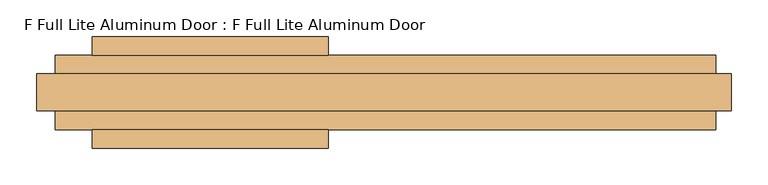
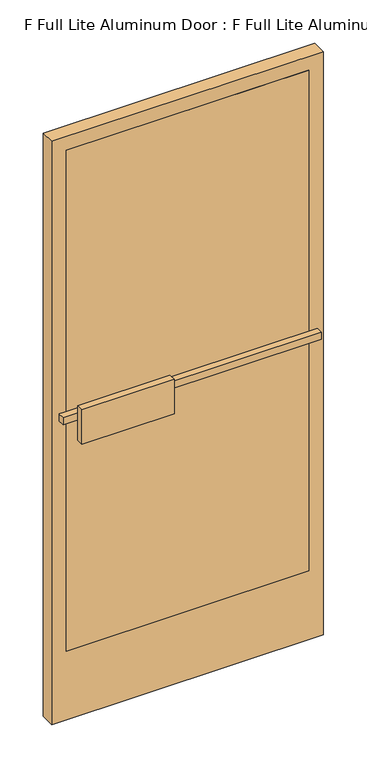
"""IFC4 building model written with IfcOpenShell, lengths in millimetres: door geometry, F Full Lite Aluminum Door : F Full Lite Aluminum Door."""

from ifc_helpers import new_model, si_unit, frame, origin, place, context, project, spatial, polyline, outline, extrude, source, transform, mapped, element, save


def f_full_lite_aluminum_door_f_full_lite_aluminum_door_7a9541b3(model_context):
    return source(origin(), model_context, "Body", "SweptSolid", [
        extrude(outline(polyline([(424.259375, 0.0), (-424.259375, 0.0), (-424.259375, 50.8), (424.259375, 50.8), (424.259375, 0.0)])), frame((0.0, 0.0, 254.0), z_axis=(0.0, 0.0, 1.0), x_axis=(1.0, 0.0, 0.0)), (0.0, 0.0, 1.0), 1852.6125),
        extrude(outline(polyline([(2157.4125, -475.059375), (0.0, -475.059375), (0.0, 475.059375), (2157.4125, 475.059375), (2157.4125, -475.059375)]), holes=[polyline([(2106.6125, -424.259375), (2106.6125, 424.259375), (254.0, 424.259375), (254.0, -424.259375), (2106.6125, -424.259375)])]), frame((0.0, 0.0, 0.0), z_axis=(0.0, 1.0, 0.0), x_axis=(0.0, 0.0, 1.0)), (0.0, 0.0, 1.0), 50.8),
        extrude(outline(polyline([(-398.859375, -25.4), (-76.2, -25.4), (-76.2, -50.8), (-398.859375, -50.8), (-398.859375, -25.4)])), frame((0.0, 0.0, 1041.4), z_axis=(0.0, 0.0, 1.0), x_axis=(1.0, 0.0, 0.0)), (0.0, 0.0, 1.0), 127.0),
        extrude(outline(polyline([(-76.2, 76.2), (-398.859375, 76.2), (-398.859375, 101.6), (-76.2, 101.6), (-76.2, 76.2)])), frame((0.0, 0.0, 1065.2125), z_axis=(0.0, 0.0, 1.0), x_axis=(1.0, 0.0, 0.0)), (0.0, 0.0, 1.0), 127.0),
        extrude(outline(polyline([(-449.659375, 0.0), (453.2879464, 0.0), (453.2879464, -25.4), (-449.659375, -25.4), (-449.659375, 0.0)])), frame((0.0, 0.0, 1116.0125), z_axis=(0.0, 0.0, 1.0), x_axis=(1.0, 0.0, 0.0)), (0.0, 0.0, 1.0), 25.4),
        extrude(outline(polyline([(453.2879464, 50.8), (-449.659375, 50.8), (-449.659375, 76.2), (453.2879464, 76.2), (453.2879464, 50.8)])), frame((0.0, 0.0, 1092.2), z_axis=(0.0, 0.0, 1.0), x_axis=(1.0, 0.0, 0.0)), (0.0, 0.0, 1.0), 25.4),
    ])


if __name__ == "__main__":
    model = new_model("IFC4")
    model_context = context("Model", 3, world=origin())
    ifc_project = project(units=[si_unit("LENGTHUNIT", "METRE", prefix="MILLI")], contexts=[model_context])
    site = spatial("IfcSite", under=ifc_project)
    building = spatial("IfcBuilding", under=site)
    placement = place(None, origin())
    f_full_lite_aluminum_door_f_full_lite_aluminum_door_shape = f_full_lite_aluminum_door_f_full_lite_aluminum_door_7a9541b3(model_context)
    element("IfcDoor", 1, ObjectType="F Full Lite Aluminum Door : F Full Lite Aluminum Door", at=placement, inside=building, context=model_context, shape_type="MappedRepresentation", body=[
        mapped(f_full_lite_aluminum_door_f_full_lite_aluminum_door_shape, transform((0.0, 0.0, 0.0), x_axis=(1.0, 0.0, 0.0), y_axis=(0.0, 1.0, 0.0), z_axis=(0.0, 0.0, 1.0))),
    ])
    save(model, "model.ifc")

# Revit data of these elements
# Type "F Full Lite Aluminum Door : F Full Lite Aluminum Door"
#   Type Mark = "20"
#   Construction Type Id = "SGL"
#   Assembly Code = "B2030100"
#   Analytic Construction = "Large single-glazed windows"
#   Visual Light Transmittance = 0.9
#   Thermal Resistance (R) = 0.179801 (m²·K)/W
#   Solar Heat Gain Coefficient = 0.86
#   Heat Transfer Coefficient (U) = 5.5617 W/(m²·K)
#   Offset = 0' - 2"
#   Function = 1
#   Handle Material = Aluminum
#   Glazing Material = Glass
# Element 1 (IfcDoor, "F Full Lite Aluminum Door : F Full Lite Aluminum Door")
#   Materials on its faces: "Aluminum", "Glass"
# Materials
#   "Aluminum": class "Metal", colour RGB 247 247 247, transparency 0, Description = "Aluminum 6061", Cost = 0
#   "Glass": class "Unassigned", colour RGB 0 0 255, transparency 0.75
